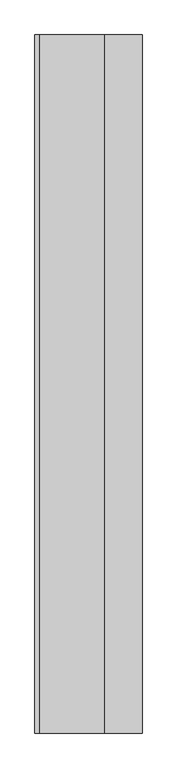
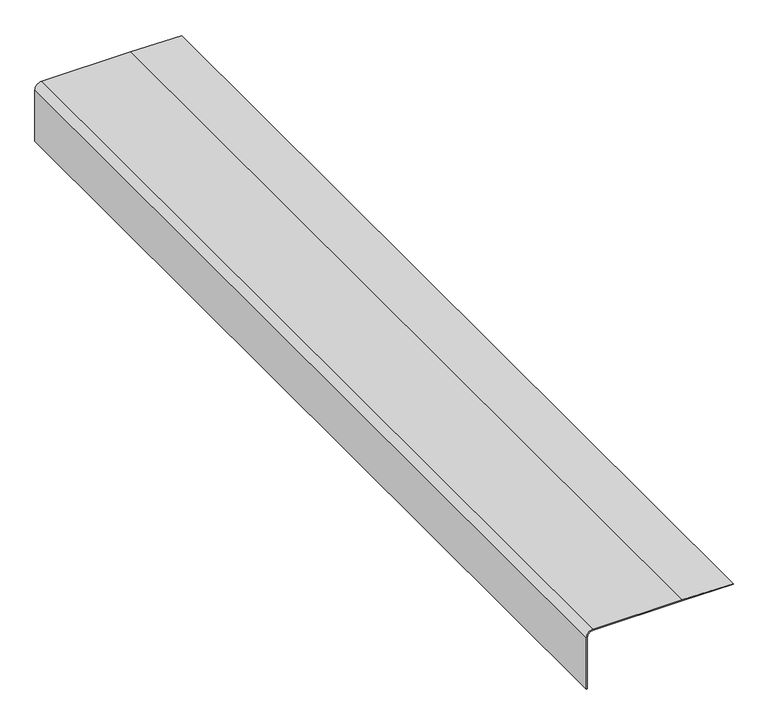
"""IFC4 building model written with IfcOpenShell, lengths in millimetres: proxy geometry, Membrane060 15930 : Membrane060 15930."""

import ifcopenshell
import ifcopenshell.guid

model = None  # the IFC model being written
_history = None  # IfcOwnerHistory: only IFC2X3 demands one
_inside = {}  # id of a spatial element -> (the spatial element, [elements in it])
_under = {}  # id of a project, library or spatial element -> (it, [spatial elements below it])
_declared = {}  # id of a project -> (the project, [libraries it declares])
_typed = {}  # id of a type object -> (the type object, [elements of that type])
_made_of = {}  # id of a material, layer set ... -> (it, [elements and type objects made of it])


def new_model(schema):
    """Start an empty IFC model of exactly this schema.

    Asked for "IFC4X3", IfcOpenShell would pick the latest addendum, in which some entities
    have other attributes; the version numbers below select the first issue.
    IFC2X3 requires an IfcOwnerHistory on every rooted entity: one is made here for all.
    """
    global model, _history
    if schema == "IFC4X3":
        model = ifcopenshell.file(schema_version=(4, 3, 0, 0))
    else:
        model = ifcopenshell.file(schema=schema)
    _inside.clear()
    _under.clear()
    _declared.clear()
    _typed.clear()
    _made_of.clear()
    _history = None
    if model.schema == "IFC2X3":
        org = make("IfcOrganization", Name="unknown")
        user = make(
            "IfcPersonAndOrganization",
            ThePerson=make("IfcPerson", FamilyName="unknown"),
            TheOrganization=org,
        )
        app = make(
            "IfcApplication",
            ApplicationDeveloper=org,
            Version="unknown",
            ApplicationFullName="unknown",
            ApplicationIdentifier="unknown",
        )
        _history = make(
            "IfcOwnerHistory",
            OwningUser=user,
            OwningApplication=app,
            ChangeAction="ADDED",
            CreationDate=0,
        )
    return model


def make(cls, **values):
    """One entity of the class cls with the attributes given. An attribute that is None is left unset."""
    return model.create_entity(
        cls, **{name: value for name, value in values.items() if value is not None}
    )


def rooted(cls, **values):
    """An entity with a GlobalId (a new one), such as an element, a storey or a relation."""
    return make(cls, GlobalId=ifcopenshell.guid.new(), OwnerHistory=_history, **values)


def si_unit(unit_type, name, prefix=None):
    """IfcSIUnit, for example si_unit("LENGTHUNIT", "METRE", prefix="MILLI")."""
    return make("IfcSIUnit", UnitType=unit_type, Prefix=prefix, Name=name)


def assignment(units):
    """IfcUnitAssignment: the units of a project."""
    return None if units is None else make("IfcUnitAssignment", Units=units)


def point(xyz):
    """IfcCartesianPoint."""
    return None if xyz is None else make("IfcCartesianPoint", Coordinates=xyz)


def direction(xyz):
    """IfcDirection."""
    return None if xyz is None else make("IfcDirection", DirectionRatios=xyz)


def frame(location, z_axis=None, x_axis=None):
    """IfcAxis2Placement3D, a coordinate frame: its origin and axes. An axis left out is left unset."""
    return make(
        "IfcAxis2Placement3D",
        Location=point(location),
        Axis=direction(z_axis),
        RefDirection=direction(x_axis),
    )


def frame_2d(location, x_axis=None):
    """IfcAxis2Placement2D, a coordinate frame in the plane: its origin and x axis."""
    return make(
        "IfcAxis2Placement2D", Location=point(location), RefDirection=direction(x_axis)
    )


def origin():
    """The frame at (0, 0, 0) with its axes left unset."""
    return frame((0.0, 0.0, 0.0))


def place(relative_to, where):
    """IfcLocalPlacement: puts the frame where relative to a parent placement (None: the world)."""
    return make(
        "IfcLocalPlacement", PlacementRelTo=relative_to, RelativePlacement=where
    )


def context(
    kind, dimensions, precision=None, world=None, true_north=None, identifier=None
):
    """IfcGeometricRepresentationContext, for example the 3D "Model" context."""
    return make(
        "IfcGeometricRepresentationContext",
        ContextIdentifier=identifier,
        ContextType=kind,
        CoordinateSpaceDimension=dimensions,
        Precision=precision,
        WorldCoordinateSystem=world,
        TrueNorth=true_north,
    )


def project(units=None, contexts=None):
    """IfcProject with its units and contexts."""
    return rooted(
        "IfcProject",
        Name="project",
        RepresentationContexts=contexts,
        UnitsInContext=assignment(units),
    )


def spatial(cls, under=None, at=None, **own):
    """A site, building, storey or space (cls), placed at a placement, below another one or the project."""
    s = rooted(cls, ObjectPlacement=at, **own)
    if under is not None:
        _under.setdefault(under.id(), (under, []))[1].append(s)
    return s


def polyline(points):
    """IfcPolyline through the points."""
    return make("IfcPolyline", Points=[point(p) for p in points])


def circle_curve(where, radius):
    """IfcCircle in the frame where."""
    return make("IfcCircle", Position=where, Radius=radius)


def trimmed(basis, trim1, trim2, sense, master):
    """IfcTrimmedCurve: the piece of a basis curve between two trims."""
    return make(
        "IfcTrimmedCurve",
        BasisCurve=basis,
        Trim1=trim1,
        Trim2=trim2,
        SenseAgreement=sense,
        MasterRepresentation=master,
    )


def segment(curve, same_sense, transition):
    """IfcCompositeCurveSegment."""
    return make(
        "IfcCompositeCurveSegment",
        Transition=transition,
        SameSense=same_sense,
        ParentCurve=curve,
    )


def composite_curve(segments, self_intersect=None):
    """IfcCompositeCurve: segments joined end to end."""
    return make("IfcCompositeCurve", Segments=segments, SelfIntersect=self_intersect)


def outline(outer, holes=None, kind="AREA"):
    """IfcArbitraryClosedProfileDef: a profile drawn as a closed curve; with holes, ...WithVoids."""
    if holes is None:
        return make("IfcArbitraryClosedProfileDef", ProfileType=kind, OuterCurve=outer)
    return make(
        "IfcArbitraryProfileDefWithVoids",
        ProfileType=kind,
        OuterCurve=outer,
        InnerCurves=holes,
    )


def extrude(swept, where, along, depth):
    """IfcExtrudedAreaSolid: the profile swept, set in the frame where, extruded along a direction by depth."""
    return make(
        "IfcExtrudedAreaSolid",
        SweptArea=swept,
        Position=where,
        ExtrudedDirection=direction(along),
        Depth=depth,
    )


def shape(context_of_items, identifier, shape_type, items):
    """IfcShapeRepresentation: the items that make up one representation, for example the "Body"."""
    return make(
        "IfcShapeRepresentation",
        ContextOfItems=context_of_items,
        RepresentationIdentifier=identifier,
        RepresentationType=shape_type,
        Items=items,
    )


def source(mapping_origin, context_of_items, identifier, shape_type, items):
    """IfcRepresentationMap: a shape defined once, which mapped items show again and again."""
    return make(
        "IfcRepresentationMap",
        MappingOrigin=mapping_origin,
        MappedRepresentation=shape(context_of_items, identifier, shape_type, items),
    )


def transform(
    local_origin,
    x_axis=None,
    y_axis=None,
    z_axis=None,
    scale=None,
    scale2=None,
    scale3=None,
    uniform=True,
):
    """IfcCartesianTransformationOperator3D, or its non-uniform kind. x_axis, y_axis, z_axis: its Axis1, 2, 3."""
    if uniform:
        return make(
            "IfcCartesianTransformationOperator3D",
            Axis1=direction(x_axis),
            Axis2=direction(y_axis),
            LocalOrigin=point(local_origin),
            Scale=scale,
            Axis3=direction(z_axis),
        )
    return make(
        "IfcCartesianTransformationOperator3DnonUniform",
        Axis1=direction(x_axis),
        Axis2=direction(y_axis),
        LocalOrigin=point(local_origin),
        Scale=scale,
        Axis3=direction(z_axis),
        Scale2=scale2,
        Scale3=scale3,
    )


def mapped(mapping_source, mapping_target):
    """IfcMappedItem: shows the shape of a source again, moved by a transform."""
    return make(
        "IfcMappedItem", MappingSource=mapping_source, MappingTarget=mapping_target
    )


def made_of(thing, what):
    """Note that an element or type object is made of a material, layer set ...; save() writes the relation."""
    if what is not None:
        _made_of.setdefault(what.id(), (what, []))[1].append(thing)
    return thing


def element(
    cls,
    number,
    at=None,
    inside=None,
    cuts=None,
    type_object=None,
    material=None,
    context=None,
    identifier="Body",
    shape_type=None,
    held_by="IfcProductDefinitionShape",
    body=None,
    shapes=None,
    **own,
):
    """One element of the class cls, such as IfcWall. Its Tag is "e" and its number.

    at: its placement. inside: the storey or other place that contains it. cuts: it is an
    opening in that element (IfcRelVoidsElement). A single representation is given by context,
    identifier, shape_type and body (its items); several are given by shapes. held_by: the class
    of the entity that holds the representations. save() writes the other relations.
    """
    e = rooted(cls, Tag="e%d" % number, ObjectPlacement=at, **own)
    if body is not None:
        shapes = [shape(context, identifier, shape_type, body)]
    if shapes is not None:
        e.Representation = make(held_by, Representations=shapes)
    if inside is not None:
        _inside.setdefault(inside.id(), (inside, []))[1].append(e)
    if cuts is not None:
        rooted(
            "IfcRelVoidsElement", RelatingBuildingElement=cuts, RelatedOpeningElement=e
        )
    if type_object is not None:
        _typed.setdefault(type_object.id(), (type_object, []))[1].append(e)
    return made_of(e, material)


def aggregate(whole, parts):
    """IfcRelAggregates: a whole, such as a stair, and the parts it consists of."""
    return rooted("IfcRelAggregates", RelatingObject=whole, RelatedObjects=parts)


def save(model, path):
    """Write the relations noted so far, then the file.

    IfcRelAggregates (storeys below a building ...), IfcRelContainedInSpatialStructure (elements
    in a storey), IfcRelDefinesByType, IfcRelAssociatesMaterial and IfcRelDeclares: one each for
    every whole, place, type object, material and project.
    """
    for whole, parts in _under.values():
        aggregate(whole, parts)
    for where, things in _inside.values():
        rooted(
            "IfcRelContainedInSpatialStructure",
            RelatedElements=things,
            RelatingStructure=where,
        )
    for kind, things in _typed.values():
        rooted("IfcRelDefinesByType", RelatedObjects=things, RelatingType=kind)
    for what, things in _made_of.values():
        rooted("IfcRelAssociatesMaterial", RelatedObjects=things, RelatingMaterial=what)
    for by, libraries in _declared.values():
        rooted("IfcRelDeclares", RelatingContext=by, RelatedDefinitions=libraries)
    model.write(path)


def generic_models_c6536bbc(model_context):
    return source(origin(), model_context, "Body", "SweptSolid", [
        extrude(outline(composite_curve([segment(trimmed(circle_curve(frame_2d((40234.5370749, -4992.792898)), 12.0), [point((40234.5370749, -5004.792898))], [point((40246.5370749, -4992.792898))], True, "CARTESIAN"), True, "CONTINUOUS"), segment(polyline([(40246.5370749, -4992.792898), (40246.5370749, -4806.2897295), (40245.0046252, -4699.8063764), (40247.0048323, -4699.8063764), (40248.5370749, -4806.2753388), (40248.5370749, -4992.792898)]), True, "CONTINUOUS"), segment(trimmed(circle_curve(frame_2d((40234.5370749, -4992.792898)), 14.0), [point((40248.5370749, -4992.792898))], [point((40234.5370749, -5006.792898))], False, "CARTESIAN"), True, "CONTINUOUS"), segment(polyline([(40234.5370749, -5006.792898), (40120.9129128, -5006.792898), (40120.9129128, -5004.792898), (40234.5370749, -5004.792898)]), True, "CONTINUOUS")], self_intersect=False)), frame((0.0, -1052.8906574, 0.0), z_axis=(0.0, 1.0, 0.0), x_axis=(0.0, 0.0, 1.0)), (0.0, 0.0, 1.0), 2000.0),
    ])


if __name__ == "__main__":
    model = new_model("IFC4")
    model_context = context("Model", 3, world=origin())
    ifc_project = project(units=[si_unit("LENGTHUNIT", "METRE", prefix="MILLI")], contexts=[model_context])
    site = spatial("IfcSite", under=ifc_project)
    building = spatial("IfcBuilding", under=site)
    placement = place(None, origin())
    generic_models_shape = generic_models_c6536bbc(model_context)
    element("IfcBuildingElementProxy", 1, Name="Membrane060 15930 : Membrane060 15930", ObjectType="Membrane060 15930 : Membrane060 15930", at=placement, inside=building, context=model_context, shape_type="MappedRepresentation", body=[
        mapped(generic_models_shape, transform((0.0, 0.0, 0.0), x_axis=(1.0, 0.0, 0.0), y_axis=(0.0, 1.0, 0.0), z_axis=(0.0, 0.0, 1.0))),
    ])
    save(model, "model.ifc")

# Revit data of these elements
# Type "Membrane060 15930 : Membrane060 15930"
#   NameOverride = "Membrane060"
# Element 1 (IfcBuildingElementProxy, "Membrane060 15930 : Membrane060 15930")
#   Materials on its faces: "THREE PLY BUILT UP ROOF MEMBRANE"
# Materials
#   "THREE PLY BUILT UP ROOF MEMBRANE": class "Unassigned", colour RGB 63 63 63, transparency 0
